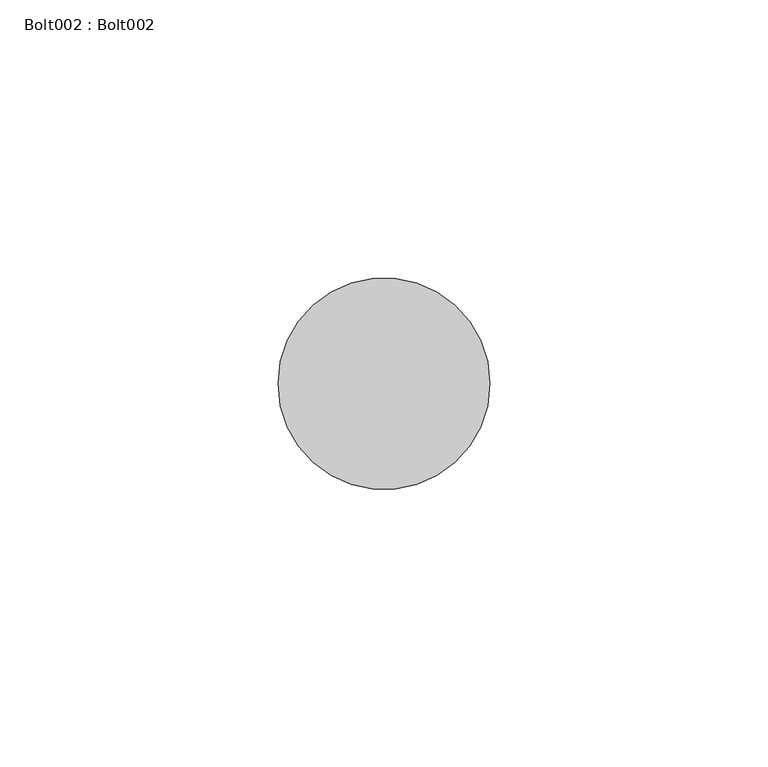
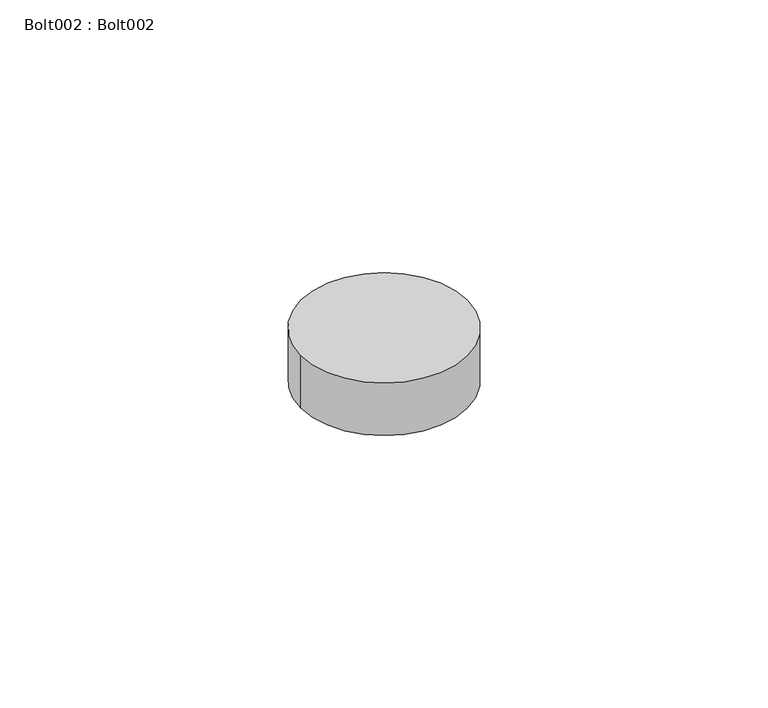
"""IFC4 building model written with IfcOpenShell, lengths in millimetres: proxy geometry, Bolt002 : Bolt002."""

from ifc_helpers import new_model, si_unit, point, frame, frame_2d, origin, place, context, project, spatial, circle_curve, trimmed, segment, composite_curve, outline, extrude, source, transform, mapped, element, save


def bolt002_bolt002_b789c14b(model_context):
    return source(origin(), model_context, "Body", "SweptSolid", [
        extrude(outline(composite_curve([segment(trimmed(circle_curve(frame_2d((7415.2612305, -1781.8449707)), 19.05), [point((7396.2112305, -1781.8449707))], [point((7434.3112305, -1781.8449707))], False, "CARTESIAN"), True, "CONTINUOUS"), segment(trimmed(circle_curve(frame_2d((7415.2612305, -1781.8449707)), 19.05), [point((7434.3112305, -1781.8449707))], [point((7396.2112305, -1781.8449707))], False, "CARTESIAN"), True, "CONTINUOUS")], self_intersect=False)), frame((0.0, 0.0, 40112.696), z_axis=(0.0, 0.0, 1.0), x_axis=(1.0, 0.0, 0.0)), (0.0, 0.0, 1.0), 12.7),
    ])


if __name__ == "__main__":
    model = new_model("IFC4")
    model_context = context("Model", 3, world=origin())
    ifc_project = project(units=[si_unit("LENGTHUNIT", "METRE", prefix="MILLI")], contexts=[model_context])
    site = spatial("IfcSite", under=ifc_project)
    building = spatial("IfcBuilding", under=site)
    placement = place(None, origin())
    bolt002_bolt002_shape = bolt002_bolt002_b789c14b(model_context)
    element("IfcBuildingElementProxy", 1, Name="Bolt002 : Bolt002", ObjectType="Bolt002 : Bolt002", at=placement, inside=building, context=model_context, shape_type="MappedRepresentation", body=[
        mapped(bolt002_bolt002_shape, transform((0.0, 0.0, 0.0), x_axis=(1.0, 0.0, 0.0), y_axis=(0.0, 1.0, 0.0), z_axis=(0.0, 0.0, 1.0))),
    ])
    save(model, "model.ifc")

# Revit data of these elements
# Type "Bolt002 : Bolt002"
#   NameOverride = "Bolt002"
# Element 1 (IfcBuildingElementProxy, "Bolt002 : Bolt002")
#   Materials on its faces: "BOLTS CONCEALED BY FLOOR FINISH"
# Materials
#   "BOLTS CONCEALED BY FLOOR FINISH": class "Unassigned", colour RGB 128 128 128, transparency 0
